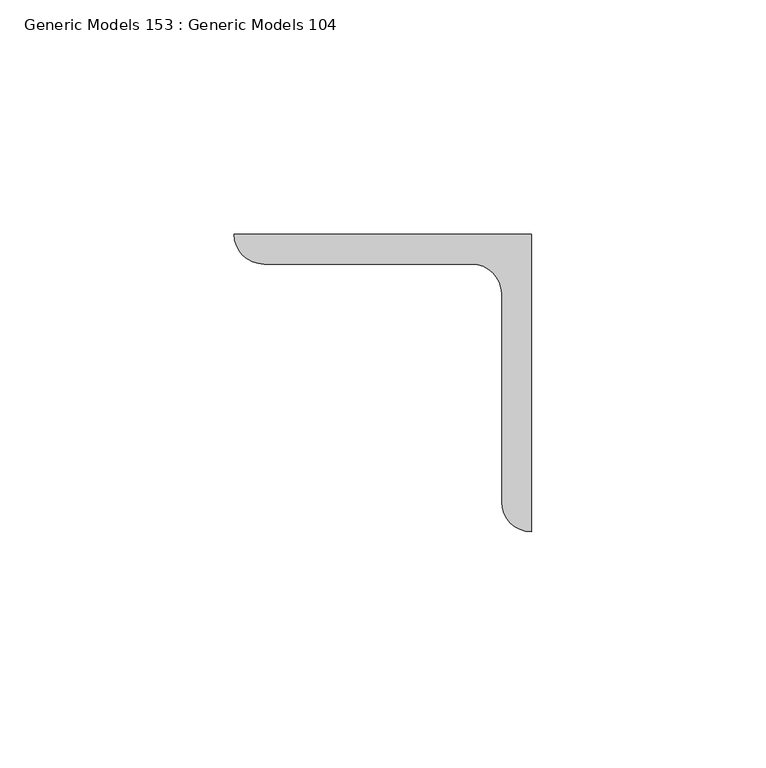
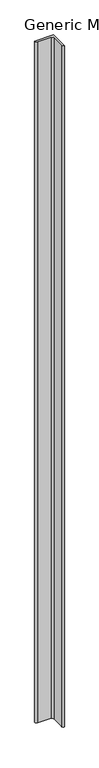
"""IFC4 building model written with IfcOpenShell, lengths in millimetres: proxy geometry, Generic Models 153 : Generic Models 104."""

from ifc_helpers import new_model, si_unit, point, frame, frame_2d, origin, place, context, project, spatial, polyline, circle_curve, trimmed, segment, composite_curve, outline, extrude, source, transform, mapped, element, save


def generic_models_153_generic_models_104_f78bf2ef(model_context):
    return source(origin(), model_context, "Body", "SweptSolid", [
        extrude(outline(composite_curve([segment(polyline([(28125.7340778, 41071.1196612), (28125.7340778, 41007.6196612)]), True, "CONTINUOUS"), segment(trimmed(circle_curve(frame_2d((28125.7340778, 41013.9696612)), 6.35), [point((28125.7340778, 41007.6196612))], [point((28119.3840778, 41013.9696612))], False, "CARTESIAN"), True, "CONTINUOUS"), segment(polyline([(28119.3840778, 41013.9696612), (28119.3840778, 41058.4196612)]), True, "CONTINUOUS"), segment(trimmed(circle_curve(frame_2d((28113.0340778, 41058.4196612)), 6.35), [point((28119.3840778, 41058.4196612))], [point((28113.0340778, 41064.7696612))], True, "CARTESIAN"), True, "CONTINUOUS"), segment(polyline([(28113.0340778, 41064.7696612), (28068.5840778, 41064.7696612)]), True, "CONTINUOUS"), segment(trimmed(circle_curve(frame_2d((28068.5840778, 41071.1196612)), 6.35), [point((28068.5840778, 41064.7696612))], [point((28062.2340778, 41071.1196612))], False, "CARTESIAN"), True, "CONTINUOUS"), segment(polyline([(28062.2340778, 41071.1196612), (28125.7340778, 41071.1196612)]), True, "CONTINUOUS")], self_intersect=False)), frame((0.0, 0.0, 266407.9), z_axis=(0.0, 0.0, 1.0), x_axis=(1.0, 0.0, 0.0)), (0.0, 0.0, 1.0), 2432.1044757),
    ])


if __name__ == "__main__":
    model = new_model("IFC4")
    model_context = context("Model", 3, world=origin())
    ifc_project = project(units=[si_unit("LENGTHUNIT", "METRE", prefix="MILLI")], contexts=[model_context])
    site = spatial("IfcSite", under=ifc_project)
    building = spatial("IfcBuilding", under=site)
    placement = place(None, origin())
    generic_models_153_generic_models_104_shape = generic_models_153_generic_models_104_f78bf2ef(model_context)
    element("IfcBuildingElementProxy", 1, Name="Generic Models 153 : Generic Models 104", ObjectType="Generic Models 153 : Generic Models 104", at=placement, inside=building, context=model_context, shape_type="MappedRepresentation", body=[
        mapped(generic_models_153_generic_models_104_shape, transform((0.0, 0.0, 0.0), x_axis=(1.0, 0.0, 0.0), y_axis=(0.0, 1.0, 0.0), z_axis=(0.0, 0.0, 1.0))),
    ])
    save(model, "model.ifc")

# Revit data of these elements
# Element 1 (IfcBuildingElementProxy, "Generic Models 153 : Generic Models 104")
#   Materials on its faces: "(2) BACK/BACK GALVANIZED ANGLES (2) L2 1/2 X 2 1/2 X 1/4\")"
# Materials
#   "(2) BACK/BACK GALVANIZED ANGLES (2) L2 1/2 X 2 1/2 X 1/4\")": class "Unassigned", colour RGB 211 211 211, transparency 0, Cost = 0
